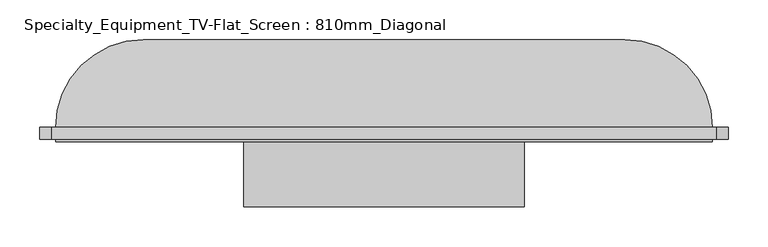
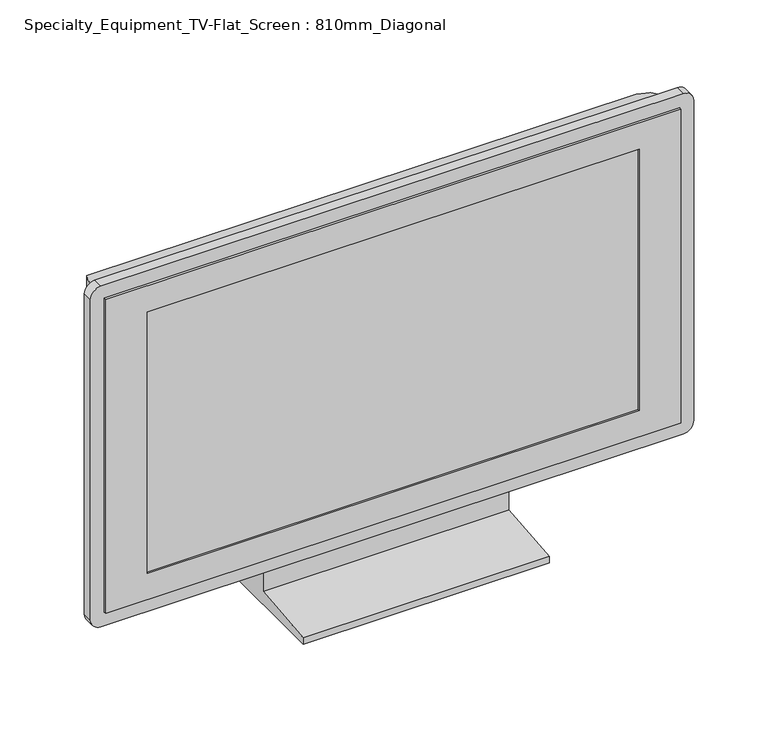
"""IFC4 building model written with IfcOpenShell, lengths in millimetres: proxy geometry, Specialty_Equipment_TV-Flat_Screen : 810mm_Diagonal."""

from ifc_helpers import new_model, si_unit, point, frame, frame_2d, origin, place, context, project, spatial, polyline, circle_curve, ellipse_curve, trimmed, segment, composite_curve, outline, extrude, faceted_brep, source, transform, mapped, element, save
from ifc_brep_helpers import plane_surface, cylinder_surface, advanced_brep


def specialty_equipment_tv_flat_screen_810mm_diagonal_56245f3a(model_context):
    return source(origin(), model_context, "Body", "SolidModel", [
        extrude(outline(polyline([(-51.4613764, 80.0), (-1.4613764, 80.0), (48.5386236, 0.0), (-151.4613764, 0.0), (-151.4613764, 10.0), (-51.4613764, 20.0), (-51.4613764, 80.0)])), frame((-180.4346678, 0.0, 0.0), z_axis=(1.0, 0.0, 0.0), x_axis=(0.0, 1.0, 0.0)), (0.0, 0.0, 1.0), 352.9803073),
        faceted_brep([(409.0357931, -69.4613764, 557.1392838), (-416.9248214, -69.4613764, 557.1392838), (-416.9248214, -69.4613764, 80.0), (409.0357931, -69.4613764, 80.0), (-356.9248214, -69.4613764, 517.1392838), (349.0357931, -69.4613764, 517.1392838), (349.0357931, -69.4613764, 120.0), (-356.9248214, -69.4613764, 120.0), (409.0357931, -51.4613764, 557.1392838), (409.0357931, -51.4613764, 80.0), (-416.9248214, -51.4613764, 80.0), (-416.9248214, -51.4613764, 557.1392838), (-356.9248214, -66.4613764, 517.1392838), (-356.9248214, -66.4613764, 120.0), (349.0357931, -66.4613764, 120.0), (349.0357931, -66.4613764, 517.1392838)], [[[0, 1, 2, 3], [4, 5, 6, 7]], [[8, 9, 10, 11]], [[1, 0, 8, 11]], [[2, 1, 11, 10]], [[3, 2, 10, 9]], [[0, 3, 9, 8]], [[12, 13, 14, 15]], [[12, 15, 5, 4]], [[15, 14, 6, 5]], [[14, 13, 7, 6]], [[13, 12, 4, 7]]]),
        extrude(outline(composite_curve([segment(polyline([(577.1392838, 414.0357931), (577.1392838, -421.9248214)]), True, "CONTINUOUS"), segment(trimmed(circle_curve(frame_2d((562.1392838, -421.9248214)), 15.0), [point((577.1392838, -421.9248214))], [point((562.1392838, -436.9248214))], False, "CARTESIAN"), True, "CONTINUOUS"), segment(polyline([(562.1392838, -436.9248214), (75.0, -436.9248214)]), True, "CONTINUOUS"), segment(trimmed(circle_curve(frame_2d((75.0, -421.9248214)), 15.0), [point((75.0, -436.9248214))], [point((60.0, -421.9248214))], False, "CARTESIAN"), True, "CONTINUOUS"), segment(polyline([(60.0, -421.9248214), (60.0, 414.0357931)]), True, "CONTINUOUS"), segment(trimmed(circle_curve(frame_2d((75.0, 414.0357931)), 15.0), [point((60.0, 414.0357931))], [point((75.0, 429.0357931))], False, "CARTESIAN"), True, "CONTINUOUS"), segment(polyline([(75.0, 429.0357931), (562.1392838, 429.0357931)]), True, "CONTINUOUS"), segment(trimmed(circle_curve(frame_2d((562.1392838, 414.0357931)), 15.0), [point((562.1392838, 429.0357931))], [point((577.1392838, 414.0357931))], False, "CARTESIAN"), True, "CONTINUOUS")], self_intersect=False), holes=[polyline([(557.1392838, 409.0357931), (80.0, 409.0357931), (80.0, -416.9248214), (557.1392838, -416.9248214), (557.1392838, 409.0357931)])]), frame((0.0, -66.4613764, 0.0), z_axis=(0.0, 1.0, 0.0), x_axis=(0.0, 0.0, 1.0)), (0.0, 0.0, 1.0), 15.0),
        advanced_brep(
        [(-416.9248214, -51.4613764, 80.0), (409.0357931, -51.4613764, 80.0), (409.0357931, -51.4613764, 557.1392838), (-416.9248214, -51.4613764, 557.1392838), (299.0357931, 58.5386236, 80.0), (-306.9248214, 58.5386236, 80.0), (-306.9248214, 58.5386236, 447.1392838), (299.0357931, 58.5386236, 447.1392838)],
        [
            (0, 1),
            (1, 2),
            (2, 3),
            (3, 0),
            (4, 5),
            (5, 6),
            (6, 7),
            (7, 4),
            (0, 5, circle_curve(frame((-306.9248214, -51.4613764, 80.0), z_axis=(0.0, 0.0, -1.0), x_axis=(-1.0, 0.0, 0.0)), 110.0)),
            (4, 1, circle_curve(frame((299.0357931, -51.4613764, 80.0), z_axis=(0.0, 0.0, -1.0), x_axis=(1.0, 0.0, 0.0)), 110.0)),
            (7, 2, ellipse_curve(frame((299.0357931, -51.4613764, 447.1392838), z_axis=(0.7071067811865475, 0.0, -0.7071067811865475), x_axis=(0.7071067811865474, 0.0, 0.7071067811865476)), 155.5634919, 110.0)),
            (6, 3, ellipse_curve(frame((-306.9248214, -51.4613764, 447.1392838), z_axis=(0.7071067811865475, 0.0, 0.7071067811865475), x_axis=(-0.7071067811865476, 0.0, 0.7071067811865474)), 155.5634919, 110.0)),
        ],
        [
            plane_surface(frame((-416.9248214, -51.4613764, 557.1392838), z_axis=(0.0, -1.0, 0.0), x_axis=(-1.0, 0.0, 0.0))),
            plane_surface(frame((-416.9248214, 58.5386236, 557.1392838), z_axis=(0.0, 1.0, 0.0), x_axis=(1.0, 0.0, 0.0))),
            plane_surface(frame((-416.9248214, -51.4613764, 80.0), z_axis=(0.0, 0.0, -1.0), x_axis=(0.0, 1.0, 0.0))),
            cylinder_surface(frame((299.0357931, -51.4613764, 80.0), z_axis=(0.0, 0.0, 1.0), x_axis=(1.0, 0.0, 0.0)), 110.0),
            cylinder_surface(frame((409.0357931, -51.4613764, 447.1392838), z_axis=(-1.0, 0.0, 0.0), x_axis=(0.0, 0.0, 1.0)), 110.0),
            cylinder_surface(frame((-306.9248214, -51.4613764, 557.1392838), z_axis=(0.0, 0.0, -1.0), x_axis=(-1.0, 0.0, 0.0)), 110.0),
        ],
        [
            (0, [[1, 2, 3, 4]]),
            (1, [[5, 6, 7, 8]]),
            (2, [[-1, 9, -5, 10]]),
            (3, [[11, -2, -10, -8]]),
            (4, [[-11, -7, 12, -3]]),
            (5, [[-12, -6, -9, -4]]),
        ],
    ),
    ])


if __name__ == "__main__":
    model = new_model("IFC4")
    model_context = context("Model", 3, world=origin())
    ifc_project = project(units=[si_unit("LENGTHUNIT", "METRE", prefix="MILLI")], contexts=[model_context])
    site = spatial("IfcSite", under=ifc_project)
    building = spatial("IfcBuilding", under=site)
    placement = place(None, origin())
    specialty_equipment_tv_flat_screen_810mm_diagonal_shape = specialty_equipment_tv_flat_screen_810mm_diagonal_56245f3a(model_context)
    element("IfcBuildingElementProxy", 1, Name="Specialty_Equipment_TV-Flat_Screen : 810mm_Diagonal", ObjectType="Specialty_Equipment_TV-Flat_Screen : 810mm_Diagonal", at=placement, inside=building, context=model_context, shape_type="MappedRepresentation", body=[
        mapped(specialty_equipment_tv_flat_screen_810mm_diagonal_shape, transform((0.0, 0.0, 0.0), x_axis=(1.0, 0.0, 0.0), y_axis=(0.0, 1.0, 0.0), z_axis=(0.0, 0.0, 1.0))),
    ])
    save(model, "model.ifc")

# Revit data of these elements
# Type "Specialty_Equipment_TV-Flat_Screen : 810mm_Diagonal"
#   SinAng = 0.49 mm
#   L = 705.961 mm
#   H = 397.139 mm
#   Thickness = 110 mm
#   Diagonal = 810 mm
#   CosAng = 0.872 mm
#   Stand [instance default] = yes
# Element 1 (IfcBuildingElementProxy, "Specialty_Equipment_TV-Flat_Screen : 810mm_Diagonal")
#   Materials on its faces: "TV - Black", "TV - Glass", "TV - Screen"
# Materials
#   "TV - Black": class "Miscellaneous", colour RGB 49 49 49, transparency 0
#   "TV - Glass": class "Miscellaneous", colour RGB 157 157 157, transparency 0.9
#   "TV - Screen": class "Miscellaneous", colour RGB 0 0 0, transparency 0
